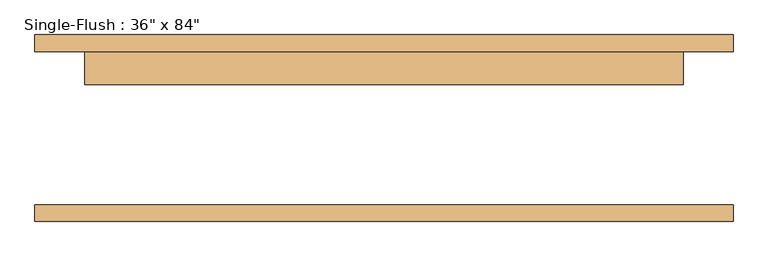
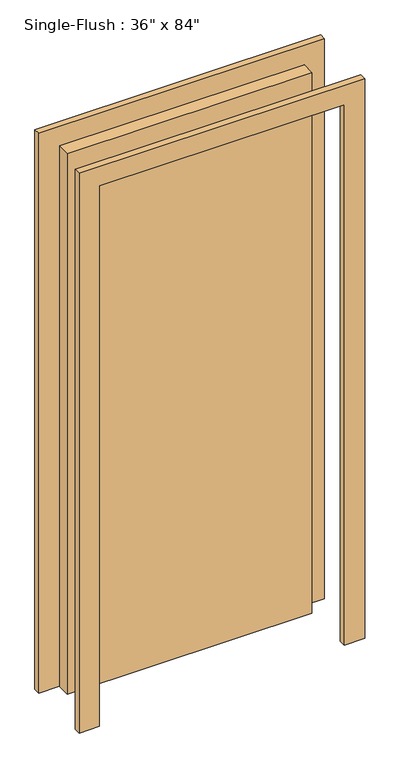
"""IFC4 building model written with IfcOpenShell, lengths in millimetres: door geometry."""

import ifcopenshell
import ifcopenshell.guid

model = None  # the IFC model being written
_history = None  # IfcOwnerHistory: only IFC2X3 demands one
_inside = {}  # id of a spatial element -> (the spatial element, [elements in it])
_under = {}  # id of a project, library or spatial element -> (it, [spatial elements below it])
_declared = {}  # id of a project -> (the project, [libraries it declares])
_typed = {}  # id of a type object -> (the type object, [elements of that type])
_made_of = {}  # id of a material, layer set ... -> (it, [elements and type objects made of it])


def new_model(schema):
    """Start an empty IFC model of exactly this schema.

    Asked for "IFC4X3", IfcOpenShell would pick the latest addendum, in which some entities
    have other attributes; the version numbers below select the first issue.
    IFC2X3 requires an IfcOwnerHistory on every rooted entity: one is made here for all.
    """
    global model, _history
    if schema == "IFC4X3":
        model = ifcopenshell.file(schema_version=(4, 3, 0, 0))
    else:
        model = ifcopenshell.file(schema=schema)
    _inside.clear()
    _under.clear()
    _declared.clear()
    _typed.clear()
    _made_of.clear()
    _history = None
    if model.schema == "IFC2X3":
        org = make("IfcOrganization", Name="unknown")
        user = make(
            "IfcPersonAndOrganization",
            ThePerson=make("IfcPerson", FamilyName="unknown"),
            TheOrganization=org,
        )
        app = make(
            "IfcApplication",
            ApplicationDeveloper=org,
            Version="unknown",
            ApplicationFullName="unknown",
            ApplicationIdentifier="unknown",
        )
        _history = make(
            "IfcOwnerHistory",
            OwningUser=user,
            OwningApplication=app,
            ChangeAction="ADDED",
            CreationDate=0,
        )
    return model


def make(cls, **values):
    """One entity of the class cls with the attributes given. An attribute that is None is left unset."""
    return model.create_entity(
        cls, **{name: value for name, value in values.items() if value is not None}
    )


def rooted(cls, **values):
    """An entity with a GlobalId (a new one), such as an element, a storey or a relation."""
    return make(cls, GlobalId=ifcopenshell.guid.new(), OwnerHistory=_history, **values)


def si_unit(unit_type, name, prefix=None):
    """IfcSIUnit, for example si_unit("LENGTHUNIT", "METRE", prefix="MILLI")."""
    return make("IfcSIUnit", UnitType=unit_type, Prefix=prefix, Name=name)


def assignment(units):
    """IfcUnitAssignment: the units of a project."""
    return None if units is None else make("IfcUnitAssignment", Units=units)


def point(xyz):
    """IfcCartesianPoint."""
    return None if xyz is None else make("IfcCartesianPoint", Coordinates=xyz)


def direction(xyz):
    """IfcDirection."""
    return None if xyz is None else make("IfcDirection", DirectionRatios=xyz)


def frame(location, z_axis=None, x_axis=None):
    """IfcAxis2Placement3D, a coordinate frame: its origin and axes. An axis left out is left unset."""
    return make(
        "IfcAxis2Placement3D",
        Location=point(location),
        Axis=direction(z_axis),
        RefDirection=direction(x_axis),
    )


def origin():
    """The frame at (0, 0, 0) with its axes left unset."""
    return frame((0.0, 0.0, 0.0))


def origin_with_axes():
    """The frame at (0, 0, 0) with the z axis (0, 0, 1) and the x axis (1, 0, 0) written out."""
    return frame((0.0, 0.0, 0.0), z_axis=(0.0, 0.0, 1.0), x_axis=(1.0, 0.0, 0.0))


def place(relative_to, where):
    """IfcLocalPlacement: puts the frame where relative to a parent placement (None: the world)."""
    return make(
        "IfcLocalPlacement", PlacementRelTo=relative_to, RelativePlacement=where
    )


def context(
    kind, dimensions, precision=None, world=None, true_north=None, identifier=None
):
    """IfcGeometricRepresentationContext, for example the 3D "Model" context."""
    return make(
        "IfcGeometricRepresentationContext",
        ContextIdentifier=identifier,
        ContextType=kind,
        CoordinateSpaceDimension=dimensions,
        Precision=precision,
        WorldCoordinateSystem=world,
        TrueNorth=true_north,
    )


def project(units=None, contexts=None):
    """IfcProject with its units and contexts."""
    return rooted(
        "IfcProject",
        Name="project",
        RepresentationContexts=contexts,
        UnitsInContext=assignment(units),
    )


def spatial(cls, under=None, at=None, **own):
    """A site, building, storey or space (cls), placed at a placement, below another one or the project."""
    s = rooted(cls, ObjectPlacement=at, **own)
    if under is not None:
        _under.setdefault(under.id(), (under, []))[1].append(s)
    return s


def polyline(points):
    """IfcPolyline through the points."""
    return make("IfcPolyline", Points=[point(p) for p in points])


def outline(outer, holes=None, kind="AREA"):
    """IfcArbitraryClosedProfileDef: a profile drawn as a closed curve; with holes, ...WithVoids."""
    if holes is None:
        return make("IfcArbitraryClosedProfileDef", ProfileType=kind, OuterCurve=outer)
    return make(
        "IfcArbitraryProfileDefWithVoids",
        ProfileType=kind,
        OuterCurve=outer,
        InnerCurves=holes,
    )


def extrude(swept, where, along, depth):
    """IfcExtrudedAreaSolid: the profile swept, set in the frame where, extruded along a direction by depth."""
    return make(
        "IfcExtrudedAreaSolid",
        SweptArea=swept,
        Position=where,
        ExtrudedDirection=direction(along),
        Depth=depth,
    )


def shape(context_of_items, identifier, shape_type, items):
    """IfcShapeRepresentation: the items that make up one representation, for example the "Body"."""
    return make(
        "IfcShapeRepresentation",
        ContextOfItems=context_of_items,
        RepresentationIdentifier=identifier,
        RepresentationType=shape_type,
        Items=items,
    )


def source(mapping_origin, context_of_items, identifier, shape_type, items):
    """IfcRepresentationMap: a shape defined once, which mapped items show again and again."""
    return make(
        "IfcRepresentationMap",
        MappingOrigin=mapping_origin,
        MappedRepresentation=shape(context_of_items, identifier, shape_type, items),
    )


def transform(
    local_origin,
    x_axis=None,
    y_axis=None,
    z_axis=None,
    scale=None,
    scale2=None,
    scale3=None,
    uniform=True,
):
    """IfcCartesianTransformationOperator3D, or its non-uniform kind. x_axis, y_axis, z_axis: its Axis1, 2, 3."""
    if uniform:
        return make(
            "IfcCartesianTransformationOperator3D",
            Axis1=direction(x_axis),
            Axis2=direction(y_axis),
            LocalOrigin=point(local_origin),
            Scale=scale,
            Axis3=direction(z_axis),
        )
    return make(
        "IfcCartesianTransformationOperator3DnonUniform",
        Axis1=direction(x_axis),
        Axis2=direction(y_axis),
        LocalOrigin=point(local_origin),
        Scale=scale,
        Axis3=direction(z_axis),
        Scale2=scale2,
        Scale3=scale3,
    )


def mapped(mapping_source, mapping_target):
    """IfcMappedItem: shows the shape of a source again, moved by a transform."""
    return make(
        "IfcMappedItem", MappingSource=mapping_source, MappingTarget=mapping_target
    )


def made_of(thing, what):
    """Note that an element or type object is made of a material, layer set ...; save() writes the relation."""
    if what is not None:
        _made_of.setdefault(what.id(), (what, []))[1].append(thing)
    return thing


def element(
    cls,
    number,
    at=None,
    inside=None,
    cuts=None,
    type_object=None,
    material=None,
    context=None,
    identifier="Body",
    shape_type=None,
    held_by="IfcProductDefinitionShape",
    body=None,
    shapes=None,
    **own,
):
    """One element of the class cls, such as IfcWall. Its Tag is "e" and its number.

    at: its placement. inside: the storey or other place that contains it. cuts: it is an
    opening in that element (IfcRelVoidsElement). A single representation is given by context,
    identifier, shape_type and body (its items); several are given by shapes. held_by: the class
    of the entity that holds the representations. save() writes the other relations.
    """
    e = rooted(cls, Tag="e%d" % number, ObjectPlacement=at, **own)
    if body is not None:
        shapes = [shape(context, identifier, shape_type, body)]
    if shapes is not None:
        e.Representation = make(held_by, Representations=shapes)
    if inside is not None:
        _inside.setdefault(inside.id(), (inside, []))[1].append(e)
    if cuts is not None:
        rooted(
            "IfcRelVoidsElement", RelatingBuildingElement=cuts, RelatedOpeningElement=e
        )
    if type_object is not None:
        _typed.setdefault(type_object.id(), (type_object, []))[1].append(e)
    return made_of(e, material)


def aggregate(whole, parts):
    """IfcRelAggregates: a whole, such as a stair, and the parts it consists of."""
    return rooted("IfcRelAggregates", RelatingObject=whole, RelatedObjects=parts)


def save(model, path):
    """Write the relations noted so far, then the file.

    IfcRelAggregates (storeys below a building ...), IfcRelContainedInSpatialStructure (elements
    in a storey), IfcRelDefinesByType, IfcRelAssociatesMaterial and IfcRelDeclares: one each for
    every whole, place, type object, material and project.
    """
    for whole, parts in _under.values():
        aggregate(whole, parts)
    for where, things in _inside.values():
        rooted(
            "IfcRelContainedInSpatialStructure",
            RelatedElements=things,
            RelatingStructure=where,
        )
    for kind, things in _typed.values():
        rooted("IfcRelDefinesByType", RelatedObjects=things, RelatingType=kind)
    for what, things in _made_of.values():
        rooted("IfcRelAssociatesMaterial", RelatedObjects=things, RelatingMaterial=what)
    for by, libraries in _declared.values():
        rooted("IfcRelDeclares", RelatingContext=by, RelatedDefinitions=libraries)
    model.write(path)


def door_10d58c7a(model_context):
    return source(origin(), model_context, "Body", "SweptSolid", [
        extrude(outline(polyline([(2209.8, -533.4), (0.0, -533.4), (0.0, -457.2), (2133.6, -457.2), (2133.6, 457.2), (0.0, 457.2), (0.0, 533.4), (2209.8, 533.4), (2209.8, -533.4)])), frame((0.0, 117.475, 0.0), z_axis=(0.0, 1.0, 0.0), x_axis=(0.0, 0.0, 1.0)), (0.0, 0.0, 1.0), 25.4),
        extrude(outline(polyline([(2209.8, 533.4), (2209.8, -533.4), (0.0, -533.4), (0.0, -457.2), (2133.6, -457.2), (2133.6, 457.2), (0.0, 457.2), (0.0, 533.4), (2209.8, 533.4)])), frame((0.0, -142.875, 0.0), z_axis=(0.0, 1.0, 0.0), x_axis=(0.0, 0.0, 1.0)), (0.0, 0.0, 1.0), 25.4),
        extrude(outline(polyline([(457.2, 66.675), (-457.2, 66.675), (-457.2, 117.475), (457.2, 117.475), (457.2, 66.675)])), origin_with_axes(), (0.0, 0.0, 1.0), 2133.6),
    ])


if __name__ == "__main__":
    model = new_model("IFC4")
    model_context = context("Model", 3, world=origin())
    ifc_project = project(units=[si_unit("LENGTHUNIT", "METRE", prefix="MILLI")], contexts=[model_context])
    site = spatial("IfcSite", under=ifc_project)
    building = spatial("IfcBuilding", under=site)
    placement = place(None, origin())
    door_shape = door_10d58c7a(model_context)
    element("IfcDoor", 1, ObjectType="Single-Flush : 36\" x 84\"", at=placement, inside=building, context=model_context, shape_type="MappedRepresentation", body=[
        mapped(door_shape, transform((0.0, 0.0, 0.0), x_axis=(1.0, 0.0, 0.0), y_axis=(0.0, 1.0, 0.0), z_axis=(0.0, 0.0, 1.0))),
    ])
    save(model, "model.ifc")

# Revit data of these elements
# Type "Single-Flush : 36\" x 84\""
#   Type Mark = "1"
#   Assembly Code = "C1020"
#   Thickness = 0' - 2"
#   Height = 7' - 0"
#   Trim Projection Ext = 0' - 1"
#   Trim Projection Int = 0' - 1"
#   Trim Width = 0' - 3"
#   Width = 3' - 0"
#   Door Material = none
#   Frame Material = none
#   Function = (empty or 0)
#   Wall Closure = (empty or 0)
